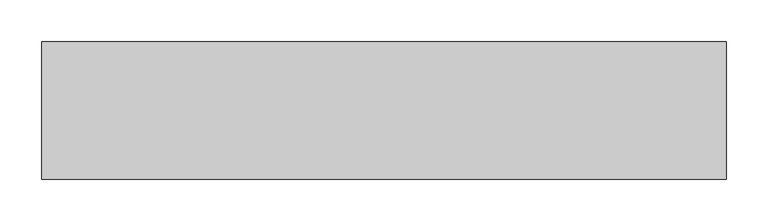
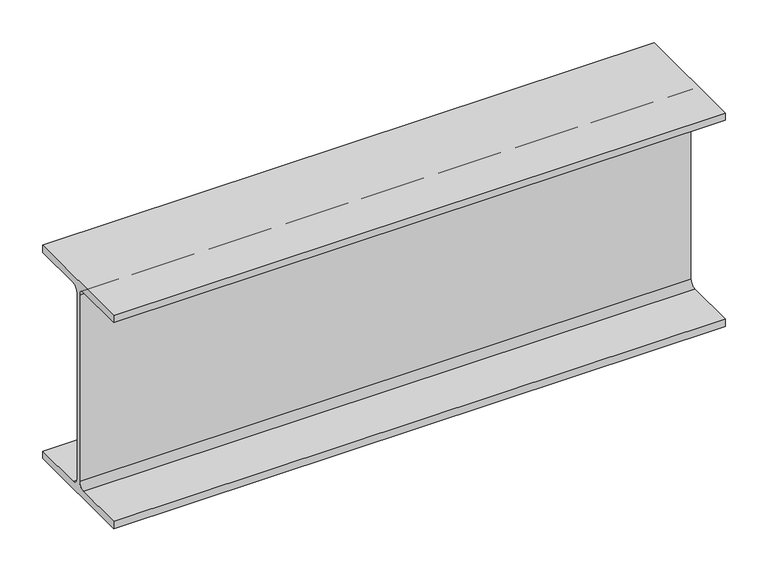
"""IFC4 building model written with IfcOpenShell, lengths in millimetres: beam geometry, Old_Steel Beam_H-KSD3502 : H_SB_ASB_H-482×300x11x15."""

from ifc_helpers import new_model, si_unit, point, frame, frame_2d, origin, place, context, project, spatial, polyline, circle_curve, trimmed, segment, composite_curve, outline, extrude, source, transform, mapped, element, save


def beam_b75d6b8e(model_context):
    return source(origin(), model_context, "Body", "SweptSolid", [
        extrude(outline(composite_curve([segment(polyline([(82.5, -141.5), (82.5, -151.7), (-82.5, -151.7), (-82.5, -141.5), (-11.9, -141.5)]), True, "CONTINUOUS"), segment(trimmed(circle_curve(frame_2d((-11.9, -132.6)), 8.9), [point((-11.9, -141.5))], [point((-3.0, -132.6))], True, "CARTESIAN"), True, "CONTINUOUS"), segment(polyline([(-3.0, -132.6), (-3.0, 132.6)]), True, "CONTINUOUS"), segment(trimmed(circle_curve(frame_2d((-11.9, 132.6)), 8.9), [point((-3.0, 132.6))], [point((-11.9, 141.5))], True, "CARTESIAN"), True, "CONTINUOUS"), segment(polyline([(-11.9, 141.5), (-82.5, 141.5), (-82.5, 151.7), (82.5, 151.7), (82.5, 141.5), (11.9, 141.5)]), True, "CONTINUOUS"), segment(trimmed(circle_curve(frame_2d((11.9, 132.6)), 8.9), [point((11.9, 141.5))], [point((3.0, 132.6))], True, "CARTESIAN"), True, "CONTINUOUS"), segment(polyline([(3.0, 132.6), (3.0, -132.6)]), True, "CONTINUOUS"), segment(trimmed(circle_curve(frame_2d((11.9, -132.6)), 8.9), [point((3.0, -132.6))], [point((11.9, -141.5))], True, "CARTESIAN"), True, "CONTINUOUS"), segment(polyline([(11.9, -141.5), (82.5, -141.5)]), True, "CONTINUOUS")], self_intersect=False)), frame((-404.8, 0.0, 0.0), z_axis=(1.0, 0.0, 0.0), x_axis=(0.0, 1.0, 0.0)), (0.0, 0.0, 1.0), 822.3),
    ])


if __name__ == "__main__":
    model = new_model("IFC4")
    model_context = context("Model", 3, world=origin())
    ifc_project = project(units=[si_unit("LENGTHUNIT", "METRE", prefix="MILLI")], contexts=[model_context])
    site = spatial("IfcSite", under=ifc_project)
    building = spatial("IfcBuilding", under=site)
    placement = place(None, origin())
    beam_shape = beam_b75d6b8e(model_context)
    element("IfcBeam", 1, ObjectType="Old_Steel Beam_H-KSD3502 : H_SB_ASB_H-482×300x11x15", at=placement, inside=building, context=model_context, shape_type="MappedRepresentation", body=[
        mapped(beam_shape, transform((0.0, 0.0, 0.0), x_axis=(1.0, 0.0, 0.0), y_axis=(0.0, 1.0, 0.0), z_axis=(0.0, 0.0, 1.0))),
    ])
    save(model, "model.ifc")

# Revit data of these elements
# Type "Old_Steel Beam_H-KSD3502 : H_SB_ASB_H-482×300x11x15"
#   Width = 30.0 cm
#   Web Thickness = 1.1 cm
#   Web Fillet = 2.6 cm
#   Warping Constant = 3680250.0 cm⁶
#   Torsional Moment of Inertia = 88.2192 cm⁴
#   Torsional Modulus = 1.0 cm³
#   Section Area = 145.5 cm²
#   Plastic Modulus weak axis = 695.0 cm³
#   Plastic Modulus strong axis = 2790.0 cm³
#   Perimeter = 2.10 m²/m
#   Nominal Weight = 114.00 kgf/m
#   Moment of Inertia weak axis = 6760.00 cm⁴
#   Moment of Inertia strong axis = 60400.00 cm⁴
#   Height = 48.2 cm
#   Flange Thickness = 1.5 cm
#   Elastic Modulus weak axis = 451.0 cm³
#   Elastic Modulus strong axis = 2500.0 cm³
#   Centroid Vertical = 24.1 cm
#   Centroid Horizontal = 15.0 cm
#   Length [instance default] = 1.5240 m
#   Structural Material [instance default] = Steel, 45-345
#   Assembly Code = ""
# Element 1 (IfcBeam, "Old_Steel Beam_H-KSD3502 : H_SB_ASB_H-482×300x11x15")
#   Structural Material = none
# Materials
#   "Steel, 45-345": class "Metal", colour RGB 189 187 185, transparency 0, Description = "Steel 345 MPa", Cost = 0
